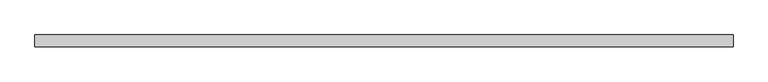
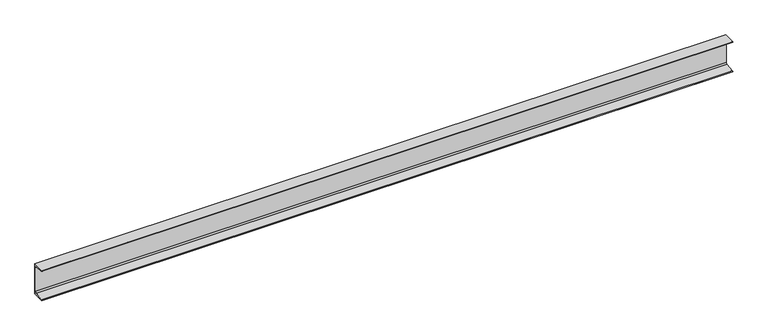
"""IFC4 building model written with IfcOpenShell, lengths in millimetres: beam geometry, C-образный профиль (ГОСТ 8240-89) Балки : [ 22."""

from ifc_helpers import new_model, si_unit, point, frame, frame_2d, origin, place, context, project, spatial, polyline, circle_curve, trimmed, segment, composite_curve, outline, extrude, source, transform, mapped, element, save


def beam_b86b2872(model_context):
    return source(origin(), model_context, "Body", "SweptSolid", [
        extrude(outline(composite_curve([segment(polyline([(22.1, 110.0), (22.1, -110.0), (-59.9, -110.0), (-59.9, -108.9686971)]), True, "CONTINUOUS"), segment(trimmed(circle_curve(frame_2d((-55.9, -108.9686971)), 4.0), [point((-59.9, -108.9686971))], [point((-56.3765809, -104.9971897))], False, "CARTESIAN"), True, "CONTINUOUS"), segment(polyline([(-56.3765809, -104.9971897), (7.8914522, -97.2850257)]), True, "CONTINUOUS"), segment(trimmed(circle_curve(frame_2d((6.7, -87.3562574)), 10.0), [point((7.8914522, -97.2850257))], [point((16.7, -87.3562574))], True, "CARTESIAN"), True, "CONTINUOUS"), segment(polyline([(16.7, -87.3562574), (16.7, 87.3562574)]), True, "CONTINUOUS"), segment(trimmed(circle_curve(frame_2d((6.7, 87.3562574)), 10.0), [point((16.7, 87.3562574))], [point((7.8914522, 97.2850257))], True, "CARTESIAN"), True, "CONTINUOUS"), segment(polyline([(7.8914522, 97.2850257), (-56.3765809, 104.9971897)]), True, "CONTINUOUS"), segment(trimmed(circle_curve(frame_2d((-55.9, 108.9686971)), 4.0), [point((-56.3765809, 104.9971897))], [point((-59.9, 108.9686971))], False, "CARTESIAN"), True, "CONTINUOUS"), segment(polyline([(-59.9, 108.9686971), (-59.9, 110.0), (22.1, 110.0)]), True, "CONTINUOUS")], self_intersect=False)), frame((-2400.0, 0.0, 0.0), z_axis=(1.0, 0.0, 0.0), x_axis=(0.0, 1.0, 0.0)), (0.0, 0.0, 1.0), 4800.0),
    ])


if __name__ == "__main__":
    model = new_model("IFC4")
    model_context = context("Model", 3, world=origin())
    ifc_project = project(units=[si_unit("LENGTHUNIT", "METRE", prefix="MILLI")], contexts=[model_context])
    site = spatial("IfcSite", under=ifc_project)
    building = spatial("IfcBuilding", under=site)
    placement = place(None, origin())
    beam_shape = beam_b86b2872(model_context)
    element("IfcBeam", 1, ObjectType="C-образный профиль (ГОСТ 8240-89) Балки : [ 22", at=placement, inside=building, context=model_context, shape_type="MappedRepresentation", body=[
        mapped(beam_shape, transform((0.0, 0.0, 0.0), x_axis=(1.0, 0.0, 0.0), y_axis=(0.0, 1.0, 0.0), z_axis=(0.0, 0.0, 1.0))),
    ])
    save(model, "model.ifc")

# Revit data of these elements
# Type "C-образный профиль (ГОСТ 8240-89) Балки : [ 22"
#   tf = 9.5 mm
#   ri = 4 mm
#   ra = 10 mm
#   W = 0.20594
#   Vz = 110 mm
#   Vy = 59.9 mm
#   Vpz = 110 mm
#   Vpy = 22.1 mm
#   Уклон = 0.12
#   Length [instance default] = 1500 mm
#   bf = 82 mm
#   d = 220 mm
#   tw = 5.4 mm
#   A = 0.00267 m²
#   Structural Material [instance default] = Металл - Сталь - 345 МПa
#   Assembly Code = ""
# Element 1 (IfcBeam, "C-образный профиль (ГОСТ 8240-89) Балки : [ 22")
#   Structural Material = C235
#   Materials on its faces: "C235"
# Materials
#   "Металл - Сталь - 345 МПa": class "Металл", colour RGB 247 247 247, transparency 0
#   "C235": class "Не назначено", colour RGB 0 0 0, transparency 0
